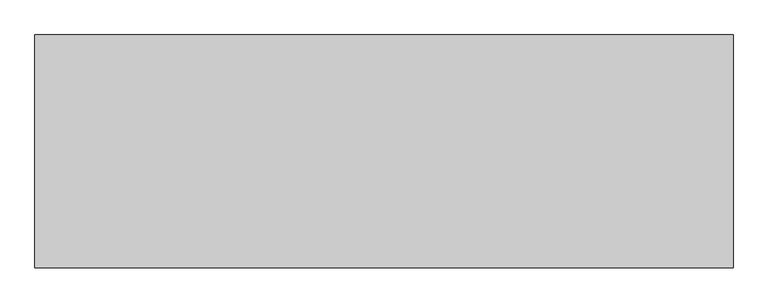
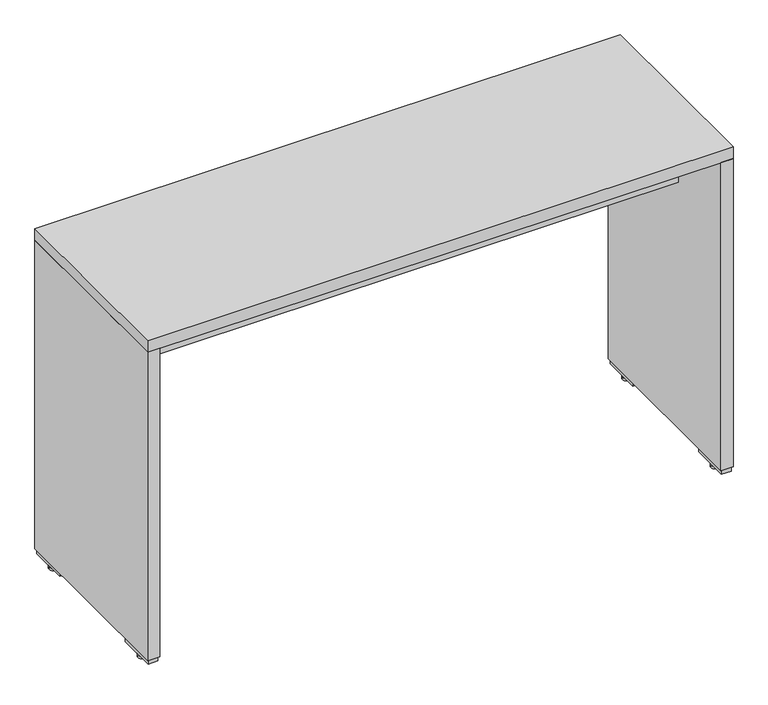
"""IFC4 building model written with IfcOpenShell, lengths in millimetres: furniture geometry, U-MCWFR67N : U-MCWFR67N."""

import ifcopenshell
import ifcopenshell.guid

model = None  # the IFC model being written
_history = None  # IfcOwnerHistory: only IFC2X3 demands one
_inside = {}  # id of a spatial element -> (the spatial element, [elements in it])
_under = {}  # id of a project, library or spatial element -> (it, [spatial elements below it])
_declared = {}  # id of a project -> (the project, [libraries it declares])
_typed = {}  # id of a type object -> (the type object, [elements of that type])
_made_of = {}  # id of a material, layer set ... -> (it, [elements and type objects made of it])


def new_model(schema):
    """Start an empty IFC model of exactly this schema.

    Asked for "IFC4X3", IfcOpenShell would pick the latest addendum, in which some entities
    have other attributes; the version numbers below select the first issue.
    IFC2X3 requires an IfcOwnerHistory on every rooted entity: one is made here for all.
    """
    global model, _history
    if schema == "IFC4X3":
        model = ifcopenshell.file(schema_version=(4, 3, 0, 0))
    else:
        model = ifcopenshell.file(schema=schema)
    _inside.clear()
    _under.clear()
    _declared.clear()
    _typed.clear()
    _made_of.clear()
    _history = None
    if model.schema == "IFC2X3":
        org = make("IfcOrganization", Name="unknown")
        user = make(
            "IfcPersonAndOrganization",
            ThePerson=make("IfcPerson", FamilyName="unknown"),
            TheOrganization=org,
        )
        app = make(
            "IfcApplication",
            ApplicationDeveloper=org,
            Version="unknown",
            ApplicationFullName="unknown",
            ApplicationIdentifier="unknown",
        )
        _history = make(
            "IfcOwnerHistory",
            OwningUser=user,
            OwningApplication=app,
            ChangeAction="ADDED",
            CreationDate=0,
        )
    return model


def make(cls, **values):
    """One entity of the class cls with the attributes given. An attribute that is None is left unset."""
    return model.create_entity(
        cls, **{name: value for name, value in values.items() if value is not None}
    )


def rooted(cls, **values):
    """An entity with a GlobalId (a new one), such as an element, a storey or a relation."""
    return make(cls, GlobalId=ifcopenshell.guid.new(), OwnerHistory=_history, **values)


def si_unit(unit_type, name, prefix=None):
    """IfcSIUnit, for example si_unit("LENGTHUNIT", "METRE", prefix="MILLI")."""
    return make("IfcSIUnit", UnitType=unit_type, Prefix=prefix, Name=name)


def assignment(units):
    """IfcUnitAssignment: the units of a project."""
    return None if units is None else make("IfcUnitAssignment", Units=units)


def point(xyz):
    """IfcCartesianPoint."""
    return None if xyz is None else make("IfcCartesianPoint", Coordinates=xyz)


def direction(xyz):
    """IfcDirection."""
    return None if xyz is None else make("IfcDirection", DirectionRatios=xyz)


def frame(location, z_axis=None, x_axis=None):
    """IfcAxis2Placement3D, a coordinate frame: its origin and axes. An axis left out is left unset."""
    return make(
        "IfcAxis2Placement3D",
        Location=point(location),
        Axis=direction(z_axis),
        RefDirection=direction(x_axis),
    )


def frame_2d(location, x_axis=None):
    """IfcAxis2Placement2D, a coordinate frame in the plane: its origin and x axis."""
    return make(
        "IfcAxis2Placement2D", Location=point(location), RefDirection=direction(x_axis)
    )


def origin():
    """The frame at (0, 0, 0) with its axes left unset."""
    return frame((0.0, 0.0, 0.0))


def origin_with_axes():
    """The frame at (0, 0, 0) with the z axis (0, 0, 1) and the x axis (1, 0, 0) written out."""
    return frame((0.0, 0.0, 0.0), z_axis=(0.0, 0.0, 1.0), x_axis=(1.0, 0.0, 0.0))


def place(relative_to, where):
    """IfcLocalPlacement: puts the frame where relative to a parent placement (None: the world)."""
    return make(
        "IfcLocalPlacement", PlacementRelTo=relative_to, RelativePlacement=where
    )


def context(
    kind, dimensions, precision=None, world=None, true_north=None, identifier=None
):
    """IfcGeometricRepresentationContext, for example the 3D "Model" context."""
    return make(
        "IfcGeometricRepresentationContext",
        ContextIdentifier=identifier,
        ContextType=kind,
        CoordinateSpaceDimension=dimensions,
        Precision=precision,
        WorldCoordinateSystem=world,
        TrueNorth=true_north,
    )


def project(units=None, contexts=None):
    """IfcProject with its units and contexts."""
    return rooted(
        "IfcProject",
        Name="project",
        RepresentationContexts=contexts,
        UnitsInContext=assignment(units),
    )


def spatial(cls, under=None, at=None, **own):
    """A site, building, storey or space (cls), placed at a placement, below another one or the project."""
    s = rooted(cls, ObjectPlacement=at, **own)
    if under is not None:
        _under.setdefault(under.id(), (under, []))[1].append(s)
    return s


def polyline(points):
    """IfcPolyline through the points."""
    return make("IfcPolyline", Points=[point(p) for p in points])


def circle_curve(where, radius):
    """IfcCircle in the frame where."""
    return make("IfcCircle", Position=where, Radius=radius)


def trimmed(basis, trim1, trim2, sense, master):
    """IfcTrimmedCurve: the piece of a basis curve between two trims."""
    return make(
        "IfcTrimmedCurve",
        BasisCurve=basis,
        Trim1=trim1,
        Trim2=trim2,
        SenseAgreement=sense,
        MasterRepresentation=master,
    )


def segment(curve, same_sense, transition):
    """IfcCompositeCurveSegment."""
    return make(
        "IfcCompositeCurveSegment",
        Transition=transition,
        SameSense=same_sense,
        ParentCurve=curve,
    )


def composite_curve(segments, self_intersect=None):
    """IfcCompositeCurve: segments joined end to end."""
    return make("IfcCompositeCurve", Segments=segments, SelfIntersect=self_intersect)


def outline(outer, holes=None, kind="AREA"):
    """IfcArbitraryClosedProfileDef: a profile drawn as a closed curve; with holes, ...WithVoids."""
    if holes is None:
        return make("IfcArbitraryClosedProfileDef", ProfileType=kind, OuterCurve=outer)
    return make(
        "IfcArbitraryProfileDefWithVoids",
        ProfileType=kind,
        OuterCurve=outer,
        InnerCurves=holes,
    )


def extrude(swept, where, along, depth):
    """IfcExtrudedAreaSolid: the profile swept, set in the frame where, extruded along a direction by depth."""
    return make(
        "IfcExtrudedAreaSolid",
        SweptArea=swept,
        Position=where,
        ExtrudedDirection=direction(along),
        Depth=depth,
    )


def shape(context_of_items, identifier, shape_type, items):
    """IfcShapeRepresentation: the items that make up one representation, for example the "Body"."""
    return make(
        "IfcShapeRepresentation",
        ContextOfItems=context_of_items,
        RepresentationIdentifier=identifier,
        RepresentationType=shape_type,
        Items=items,
    )


def source(mapping_origin, context_of_items, identifier, shape_type, items):
    """IfcRepresentationMap: a shape defined once, which mapped items show again and again."""
    return make(
        "IfcRepresentationMap",
        MappingOrigin=mapping_origin,
        MappedRepresentation=shape(context_of_items, identifier, shape_type, items),
    )


def transform(
    local_origin,
    x_axis=None,
    y_axis=None,
    z_axis=None,
    scale=None,
    scale2=None,
    scale3=None,
    uniform=True,
):
    """IfcCartesianTransformationOperator3D, or its non-uniform kind. x_axis, y_axis, z_axis: its Axis1, 2, 3."""
    if uniform:
        return make(
            "IfcCartesianTransformationOperator3D",
            Axis1=direction(x_axis),
            Axis2=direction(y_axis),
            LocalOrigin=point(local_origin),
            Scale=scale,
            Axis3=direction(z_axis),
        )
    return make(
        "IfcCartesianTransformationOperator3DnonUniform",
        Axis1=direction(x_axis),
        Axis2=direction(y_axis),
        LocalOrigin=point(local_origin),
        Scale=scale,
        Axis3=direction(z_axis),
        Scale2=scale2,
        Scale3=scale3,
    )


def mapped(mapping_source, mapping_target):
    """IfcMappedItem: shows the shape of a source again, moved by a transform."""
    return make(
        "IfcMappedItem", MappingSource=mapping_source, MappingTarget=mapping_target
    )


def made_of(thing, what):
    """Note that an element or type object is made of a material, layer set ...; save() writes the relation."""
    if what is not None:
        _made_of.setdefault(what.id(), (what, []))[1].append(thing)
    return thing


def element(
    cls,
    number,
    at=None,
    inside=None,
    cuts=None,
    type_object=None,
    material=None,
    context=None,
    identifier="Body",
    shape_type=None,
    held_by="IfcProductDefinitionShape",
    body=None,
    shapes=None,
    **own,
):
    """One element of the class cls, such as IfcWall. Its Tag is "e" and its number.

    at: its placement. inside: the storey or other place that contains it. cuts: it is an
    opening in that element (IfcRelVoidsElement). A single representation is given by context,
    identifier, shape_type and body (its items); several are given by shapes. held_by: the class
    of the entity that holds the representations. save() writes the other relations.
    """
    e = rooted(cls, Tag="e%d" % number, ObjectPlacement=at, **own)
    if body is not None:
        shapes = [shape(context, identifier, shape_type, body)]
    if shapes is not None:
        e.Representation = make(held_by, Representations=shapes)
    if inside is not None:
        _inside.setdefault(inside.id(), (inside, []))[1].append(e)
    if cuts is not None:
        rooted(
            "IfcRelVoidsElement", RelatingBuildingElement=cuts, RelatedOpeningElement=e
        )
    if type_object is not None:
        _typed.setdefault(type_object.id(), (type_object, []))[1].append(e)
    return made_of(e, material)


def aggregate(whole, parts):
    """IfcRelAggregates: a whole, such as a stair, and the parts it consists of."""
    return rooted("IfcRelAggregates", RelatingObject=whole, RelatedObjects=parts)


def save(model, path):
    """Write the relations noted so far, then the file.

    IfcRelAggregates (storeys below a building ...), IfcRelContainedInSpatialStructure (elements
    in a storey), IfcRelDefinesByType, IfcRelAssociatesMaterial and IfcRelDeclares: one each for
    every whole, place, type object, material and project.
    """
    for whole, parts in _under.values():
        aggregate(whole, parts)
    for where, things in _inside.values():
        rooted(
            "IfcRelContainedInSpatialStructure",
            RelatedElements=things,
            RelatingStructure=where,
        )
    for kind, things in _typed.values():
        rooted("IfcRelDefinesByType", RelatedObjects=things, RelatingType=kind)
    for what, things in _made_of.values():
        rooted("IfcRelAssociatesMaterial", RelatedObjects=things, RelatingMaterial=what)
    for by, libraries in _declared.values():
        rooted("IfcRelDeclares", RelatingContext=by, RelatedDefinitions=libraries)
    model.write(path)


def furniture_ebb63cec(model_context):
    return source(origin(), model_context, "Body", "SweptSolid", [
        extrude(outline(composite_curve([segment(trimmed(circle_curve(frame_2d((-881.0, -235.7499989)), 12.5), [point((-893.5, -235.7499989))], [point((-868.5, -235.7499989))], False, "CARTESIAN"), True, "CONTINUOUS"), segment(trimmed(circle_curve(frame_2d((-881.0, -235.7499989)), 12.5), [point((-868.5, -235.7499989))], [point((-893.5, -235.7499989))], False, "CARTESIAN"), True, "CONTINUOUS")], self_intersect=False)), origin_with_axes(), (0.0, 0.0, 1.0), 7.0),
        extrude(outline(composite_curve([segment(trimmed(circle_curve(frame_2d((881.0, -235.7499989)), 12.5), [point((868.5, -235.7499989))], [point((893.5, -235.7499989))], False, "CARTESIAN"), True, "CONTINUOUS"), segment(trimmed(circle_curve(frame_2d((881.0, -235.7499989)), 12.5), [point((893.5, -235.7499989))], [point((868.5, -235.7499989))], False, "CARTESIAN"), True, "CONTINUOUS")], self_intersect=False)), origin_with_axes(), (0.0, 0.0, 1.0), 7.0),
        extrude(outline(composite_curve([segment(trimmed(circle_curve(frame_2d((-881.0, 235.7499989)), 12.5), [point((-893.5, 235.7499989))], [point((-868.5, 235.7499989))], False, "CARTESIAN"), True, "CONTINUOUS"), segment(trimmed(circle_curve(frame_2d((-881.0, 235.7499989)), 12.5), [point((-868.5, 235.7499989))], [point((-893.5, 235.7499989))], False, "CARTESIAN"), True, "CONTINUOUS")], self_intersect=False)), origin_with_axes(), (0.0, 0.0, 1.0), 7.0),
        extrude(outline(composite_curve([segment(trimmed(circle_curve(frame_2d((881.0, 235.7499989)), 12.5), [point((868.5, 235.7499989))], [point((893.5, 235.7499989))], False, "CARTESIAN"), True, "CONTINUOUS"), segment(trimmed(circle_curve(frame_2d((881.0, 235.7499989)), 12.5), [point((893.5, 235.7499989))], [point((868.5, 235.7499989))], False, "CARTESIAN"), True, "CONTINUOUS")], self_intersect=False)), origin_with_axes(), (0.0, 0.0, 1.0), 7.0),
        extrude(outline(composite_curve([segment(trimmed(circle_curve(frame_2d((-881.0, -235.7499989)), 4.0), [point((-885.0, -235.7499989))], [point((-877.0, -235.7499989))], False, "CARTESIAN"), True, "CONTINUOUS"), segment(trimmed(circle_curve(frame_2d((-881.0, -235.7499989)), 4.0), [point((-877.0, -235.7499989))], [point((-885.0, -235.7499989))], False, "CARTESIAN"), True, "CONTINUOUS")], self_intersect=False)), frame((0.0, 0.0, 7.0), z_axis=(0.0, 0.0, 1.0), x_axis=(1.0, 0.0, 0.0)), (0.0, 0.0, 1.0), 8.0),
        extrude(outline(composite_curve([segment(trimmed(circle_curve(frame_2d((-881.0, 235.7499989)), 4.0), [point((-885.0, 235.7499989))], [point((-877.0, 235.7499989))], False, "CARTESIAN"), True, "CONTINUOUS"), segment(trimmed(circle_curve(frame_2d((-881.0, 235.7499989)), 4.0), [point((-877.0, 235.7499989))], [point((-885.0, 235.7499989))], False, "CARTESIAN"), True, "CONTINUOUS")], self_intersect=False)), frame((0.0, 0.0, 7.0), z_axis=(0.0, 0.0, 1.0), x_axis=(1.0, 0.0, 0.0)), (0.0, 0.0, 1.0), 8.0),
        extrude(outline(composite_curve([segment(trimmed(circle_curve(frame_2d((881.0, -235.7499989)), 4.0), [point((877.0, -235.7499989))], [point((885.0, -235.7499989))], False, "CARTESIAN"), True, "CONTINUOUS"), segment(trimmed(circle_curve(frame_2d((881.0, -235.7499989)), 4.0), [point((885.0, -235.7499989))], [point((877.0, -235.7499989))], False, "CARTESIAN"), True, "CONTINUOUS")], self_intersect=False)), frame((0.0, 0.0, 7.0), z_axis=(0.0, 0.0, 1.0), x_axis=(1.0, 0.0, 0.0)), (0.0, 0.0, 1.0), 8.0),
        extrude(outline(composite_curve([segment(trimmed(circle_curve(frame_2d((881.0, 235.7499989)), 4.0), [point((877.0, 235.7499989))], [point((885.0, 235.7499989))], False, "CARTESIAN"), True, "CONTINUOUS"), segment(trimmed(circle_curve(frame_2d((881.0, 235.7499989)), 4.0), [point((885.0, 235.7499989))], [point((877.0, 235.7499989))], False, "CARTESIAN"), True, "CONTINUOUS")], self_intersect=False)), frame((0.0, 0.0, 7.0), z_axis=(0.0, 0.0, 1.0), x_axis=(1.0, 0.0, 0.0)), (0.0, 0.0, 1.0), 8.0),
        extrude(outline(polyline([(-896.0, -175.3999989), (-866.0, -175.3999989), (-866.0, -296.0999989), (-896.0, -296.0999989), (-896.0, -175.3999989)])), frame((0.0, 0.0, 15.0), z_axis=(0.0, 0.0, 1.0), x_axis=(1.0, 0.0, 0.0)), (0.0, 0.0, 1.0), 15.0),
        extrude(outline(polyline([(896.0, -175.3999989), (896.0, -296.0999989), (866.0, -296.0999989), (866.0, -175.3999989), (896.0, -175.3999989)])), frame((0.0, 0.0, 15.0), z_axis=(0.0, 0.0, 1.0), x_axis=(1.0, 0.0, 0.0)), (0.0, 0.0, 1.0), 15.0),
        extrude(outline(polyline([(-896.0, 175.3999989), (-896.0, 296.0999989), (-866.0, 296.0999989), (-866.0, 175.3999989), (-896.0, 175.3999989)])), frame((0.0, 0.0, 15.0), z_axis=(0.0, 0.0, 1.0), x_axis=(1.0, 0.0, 0.0)), (0.0, 0.0, 1.0), 15.0),
        extrude(outline(polyline([(896.0, 175.3999989), (866.0, 175.3999989), (866.0, 296.0999989), (896.0, 296.0999989), (896.0, 175.3999989)])), frame((0.0, 0.0, 15.0), z_axis=(0.0, 0.0, 1.0), x_axis=(1.0, 0.0, 0.0)), (0.0, 0.0, 1.0), 15.0),
        extrude(outline(polyline([(862.0, 38.8370388), (-862.0, 38.8370388), (-862.0, 74.9), (862.0, 74.9), (862.0, 38.8370388)])), frame((0.0, 0.0, 832.0000577), z_axis=(0.0, 0.0, 1.0), x_axis=(1.0, 0.0, 0.0)), (0.0, 0.0, 1.0), 199.9999423),
        extrude(outline(polyline([(862.0, -38.8370388), (862.0, -74.9), (-862.0, -74.9), (-862.0, -38.8370388), (862.0, -38.8370388)])), frame((0.0, 0.0, 832.0000577), z_axis=(0.0, 0.0, 1.0), x_axis=(1.0, 0.0, 0.0)), (0.0, 0.0, 1.0), 199.9999423),
        extrude(outline(polyline([(30.6, -900.0), (30.0, -899.4), (30.0, -862.5034598), (30.6, -862.0), (1032.0, -862.0), (1032.0, -900.0), (30.6, -900.0)])), frame((0.0, -300.0, 0.0), z_axis=(0.0, 1.0, 0.0), x_axis=(0.0, 0.0, 1.0)), (0.0, 0.0, 1.0), 599.9999989),
        extrude(outline(polyline([(30.6, 900.0), (1032.0, 900.0), (1032.0, 862.0), (30.6, 862.0), (30.0, 862.5034598), (30.0, 899.4), (30.6, 900.0)])), frame((0.0, -300.0, 0.0), z_axis=(0.0, 1.0, 0.0), x_axis=(0.0, 0.0, 1.0)), (0.0, 0.0, 1.0), 599.9999989),
        extrude(outline(polyline([(900.0, 300.0), (900.0, -300.0), (-900.0, -300.0), (-900.0, 300.0), (900.0, 300.0)])), frame((0.0, 0.0, 1032.0), z_axis=(0.0, 0.0, 1.0), x_axis=(1.0, 0.0, 0.0)), (0.0, 0.0, 1.0), 38.0),
    ])


if __name__ == "__main__":
    model = new_model("IFC4")
    model_context = context("Model", 3, world=origin())
    ifc_project = project(units=[si_unit("LENGTHUNIT", "METRE", prefix="MILLI")], contexts=[model_context])
    site = spatial("IfcSite", under=ifc_project)
    building = spatial("IfcBuilding", under=site)
    placement = place(None, origin())
    furniture_shape = furniture_ebb63cec(model_context)
    element("IfcFurniture", 1, ObjectType="U-MCWFR67N : U-MCWFR67N", at=placement, inside=building, context=model_context, shape_type="MappedRepresentation", body=[
        mapped(furniture_shape, transform((0.0, 0.0, 0.0), x_axis=(1.0, 0.0, 0.0), y_axis=(0.0, 1.0, 0.0), z_axis=(0.0, 0.0, 1.0))),
    ])
    save(model, "model.ifc")

# Revit data of these elements
# Type "U-MCWFR67N : U-MCWFR67N"
#   Youtube clip = ""
#   Weight Net (kg) = ""
#   WarrantyStartDate = ""
#   WarrantyDuration = ""
#   Uniclass 2.0 Description = "Desks, Tables And Worktops"
#   Uniclass 2.0 Code = "PR-31-22"
#   Uniclass 1.4 Description = "Conference room furniture"
#   Uniclass 1.4 Code = "L8536"
#   URL = "http://kinnarps.bimobject.com/U-MCWFR67N"
#   UNSPSC Category = "Furniture and Furnishings"
#   TypeName = "U-MCWFR67N"
#   Technical description = "http://www.kinnarps.com/en/International/ProductsInspiration/Office/ConferenceTables/Product/?prodid=305786"
#   TagNumber = ""
#   Size = ""
#   SerialNumber = ""
#   Product identifier = "kinnarps.bimobject.com/U-MCWFR67N"
#   Product group = "MULTICOM"
#   Product family = "Conference tables"
#   Product data url = "http://www.kinnarps.com/en/International/ProductsInspiration/Office/ConferenceTables/Product/?prodid=305786"
#   Product SKU = "U-MCWFR67N"
#   Omniclass = "23.40.70.14.64.11"
#   NominalWidth = ""
#   NominalHeight = ""
#   Name of the object = "MULTICOM_U-MCWFR67N"
#   NBS Reference Description = "Desks, Tables And Worktops"
#   NBS Reference = "31-22"
#   Model = "MULTICOM_U-MCWFR67N"
#   Material = ""
#   Manufacturer country = "Sweden"
#   Manufacturer URL = "http://www.kinnarps.com"
#   Manufacturer = "Kinnarps"
#   InstallationDate = ""
#   Installation instructions = "http://www.kinnarps.com/en/International/ProductsInspiration/Office/ConferenceTables/Product/?prodid=305786"
#   IFC Classification = "Furniture"
#   Grade = ""
#   Finish = ""
#   Features = ""
#   Extidentifier = ""
#   Edition number = "1"
#   EAN code = ""
#   Design country = "Sweden"
#   Date of publishing = ""
#   Created on = ""
#   Created by = ""
#   ConnectionType = ""
#   Colour = ""
#   COBIe Type Category = ""
#   Barcode = ""
#   BIMobject QR code url = "http://kinnarps.bimobject.com/U-MCWFR67N"
#   BIMobject Category = "Office Furniture"
#   AssetIdentifier = ""
#   AccessibilityPerformance = ""
#   Y-Offset = 0 mm
#   Width (mm) = 1800 mm
#   X-Offset = 0 mm
#   Height (mm) = 1070 mm
#   Depth (mm) = 600 mm
#   UNSPSC Code = 56
#   Table Top [instance default] = Kinnarps-Laminate-Beech
#   Material secondary = Steel
#   Material main = Wood
#   Default Elevation = 0
# Element 1 (IfcFurniture, "U-MCWFR67N : U-MCWFR67N")
#   Table Top = Kinnarps-Laminate-White
#   Materials on its faces: "Kinnarps-Laminate-White", "Kinnarps-Plastic-Black"
# Materials
#   "Kinnarps-Laminate-Beech": class "Miscellaneous", colour RGB 174 140 106, transparency 0
#   "Steel": class "Metal", colour RGB 189 187 185, transparency 0, Cost = 0
#   "Wood": class "Miscellaneous", colour RGB 127 127 127, transparency 0
#   "Kinnarps-Laminate-White": class "Miscellaneous", colour RGB 255 255 255, transparency 0
#   "Kinnarps-Plastic-Black": class "Miscellaneous", colour RGB 0 0 0, transparency 0
